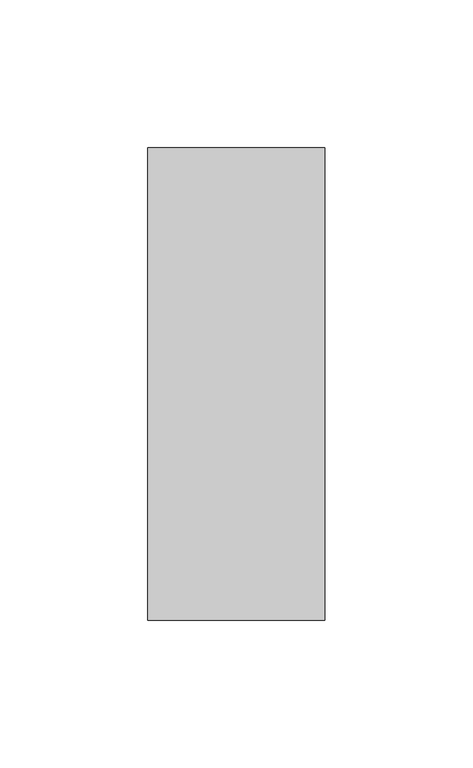
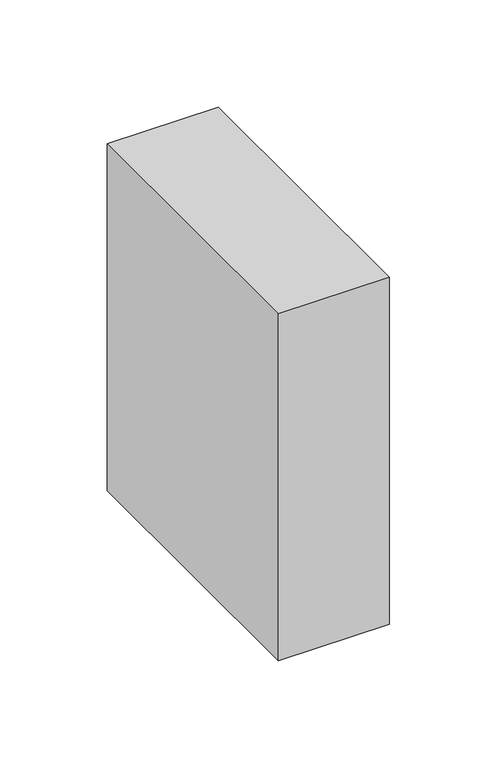
"""IFC4 building model written with IfcOpenShell, lengths in millimetres: column geometry, Madeira de lei-Coluna : Pontalete 6X16cm."""

from ifc_helpers import new_model, si_unit, frame, origin, place, context, project, spatial, polyline, outline, extrude, source, transform, mapped, element, save


def column_35730ad5(model_context):
    return source(origin(), model_context, "Body", "SweptSolid", [
        extrude(outline(polyline([(30.0, 80.0), (30.0, -80.0), (-30.0, -80.0), (-30.0, 80.0), (30.0, 80.0)])), frame((0.0, 0.0, 3110.0), z_axis=(0.0, 0.0, 1.0), x_axis=(1.0, 0.0, 0.0)), (0.0, 0.0, 1.0), 197.9),
    ])


if __name__ == "__main__":
    model = new_model("IFC4")
    model_context = context("Model", 3, world=origin())
    ifc_project = project(units=[si_unit("LENGTHUNIT", "METRE", prefix="MILLI")], contexts=[model_context])
    site = spatial("IfcSite", under=ifc_project)
    building = spatial("IfcBuilding", under=site)
    placement = place(None, origin())
    column_shape = column_35730ad5(model_context)
    element("IfcColumn", 1, ObjectType="Madeira de lei-Coluna : Pontalete 6X16cm", at=placement, inside=building, context=model_context, shape_type="MappedRepresentation", body=[
        mapped(column_shape, transform((0.0, 0.0, 0.0), x_axis=(1.0, 0.0, 0.0), y_axis=(0.0, 1.0, 0.0), z_axis=(0.0, 0.0, 1.0))),
    ])
    save(model, "model.ifc")

# Revit data of these elements
# Type "Madeira de lei-Coluna : Pontalete 6X16cm"
#   A = 0.01952 m²
#   b = 0.06 m
#   d = 0.16 m
#   Structural Material [instance default] = none
#   Assembly Code = ""
# Element 1 (IfcColumn, "Madeira de lei-Coluna : Pontalete 6X16cm")
#   Structural Material = .MADEIRAMENTO
#   Materials on its faces: ".MADEIRAMENTO"
# Materials
#   ".MADEIRAMENTO": class ".CC_MADEIRAS", colour RGB 212 179 113, transparency 0, Cost = 0
